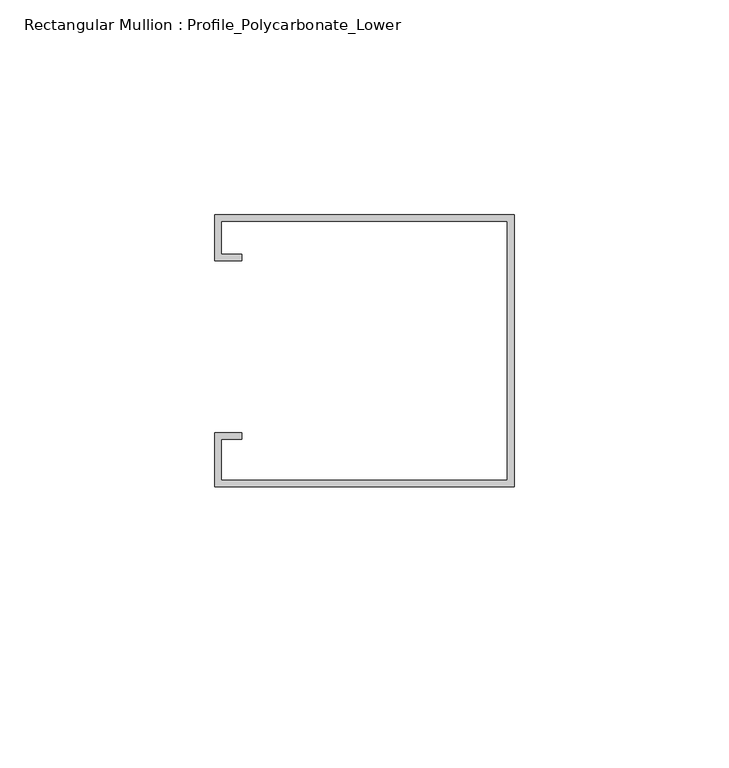
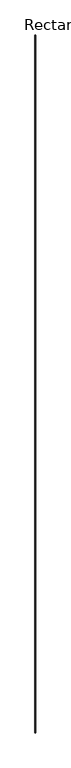
"""IFC4 building model written with IfcOpenShell, lengths in millimetres: member geometry, Rectangular Mullion : Profile_Polycarbonate_Lower."""

from ifc_helpers import new_model, si_unit, frame, origin, place, context, project, spatial, polyline, outline, extrude, source, transform, mapped, element, save


def rectangular_mullion_profile_polycarbonate_lower_cb37323c(model_context):
    return source(origin(), model_context, "Body", "SweptSolid", [
        extrude(outline(polyline([(0.0, -32.7), (-69.85, -32.7), (-69.85, -20.0), (-63.5, -20.0), (-63.5, -21.5875), (-68.2625, -21.5875), (-68.2625, -31.1125), (-1.5875, -31.1125), (-1.5875, 29.2125), (-68.2625, 29.2125), (-68.2625, 21.5875), (-63.5, 21.5875), (-63.5, 20.0), (-69.85, 20.0), (-69.85, 30.8), (0.0, 30.8), (0.0, -32.7)])), frame((0.0, 0.0, -88760.3), z_axis=(0.0, 0.0, 1.0), x_axis=(1.0, 0.0, 0.0)), (0.0, 0.0, 1.0), 88760.3),
    ])


if __name__ == "__main__":
    model = new_model("IFC4")
    model_context = context("Model", 3, world=origin())
    ifc_project = project(units=[si_unit("LENGTHUNIT", "METRE", prefix="MILLI")], contexts=[model_context])
    site = spatial("IfcSite", under=ifc_project)
    building = spatial("IfcBuilding", under=site)
    placement = place(None, origin())
    rectangular_mullion_profile_polycarbonate_lower_shape = rectangular_mullion_profile_polycarbonate_lower_cb37323c(model_context)
    element("IfcMember", 1, ObjectType="Rectangular Mullion : Profile_Polycarbonate_Lower", at=placement, inside=building, context=model_context, shape_type="MappedRepresentation", body=[
        mapped(rectangular_mullion_profile_polycarbonate_lower_shape, transform((0.0, 0.0, 0.0), x_axis=(1.0, 0.0, 0.0), y_axis=(0.0, 1.0, 0.0), z_axis=(0.0, 0.0, 1.0))),
    ])
    save(model, "model.ifc")

# Revit data of these elements
# Type "Rectangular Mullion : Profile_Polycarbonate_Lower"
#   built-in parameter 1007322 = 0.208333 (stored number, unit not read)
#   built-in parameter 1007321 = 0 (stored number, unit not read)
#   built-in parameter 1007320 = 0.00520833 (stored number, unit not read)
